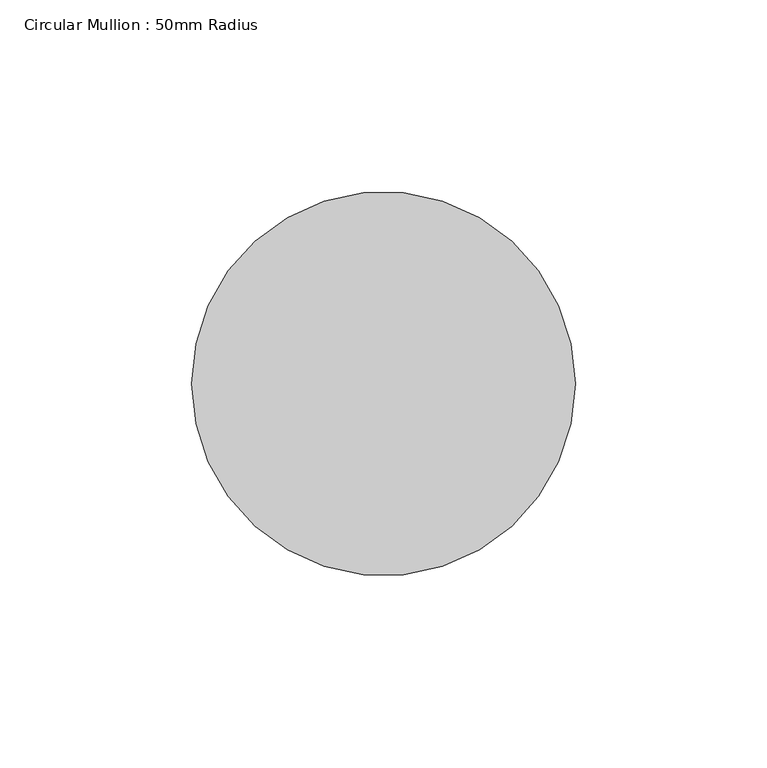
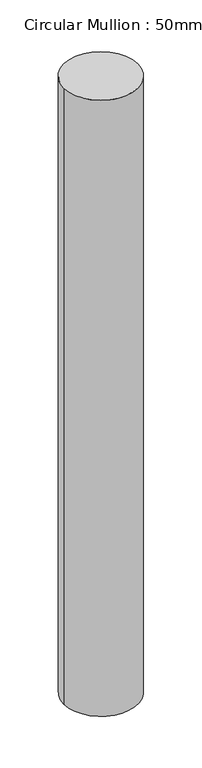
"""IFC4 building model written with IfcOpenShell, lengths in millimetres: member geometry, Circular Mullion : 50mm Radius."""

from ifc_helpers import new_model, si_unit, point, frame, origin, origin_2d, place, context, project, spatial, circle_curve, trimmed, segment, composite_curve, outline, extrude, source, transform, mapped, element, save


def circular_mullion_50mm_radius_d37bc5d8(model_context):
    return source(origin(), model_context, "Body", "SweptSolid", [
        extrude(outline(composite_curve([segment(trimmed(circle_curve(origin_2d(), 50.0), [point((50.0, 0.0))], [point((-50.0, 0.0))], False, "CARTESIAN"), True, "CONTINUOUS"), segment(trimmed(circle_curve(origin_2d(), 50.0), [point((-50.0, 0.0))], [point((50.0, 0.0))], False, "CARTESIAN"), True, "CONTINUOUS")], self_intersect=False)), frame((0.0, 0.0, -881.9892707), z_axis=(0.0, 0.0, 1.0), x_axis=(1.0, 0.0, 0.0)), (0.0, 0.0, 1.0), 881.9892707),
    ])


if __name__ == "__main__":
    model = new_model("IFC4")
    model_context = context("Model", 3, world=origin())
    ifc_project = project(units=[si_unit("LENGTHUNIT", "METRE", prefix="MILLI")], contexts=[model_context])
    site = spatial("IfcSite", under=ifc_project)
    building = spatial("IfcBuilding", under=site)
    placement = place(None, origin())
    circular_mullion_50mm_radius_shape = circular_mullion_50mm_radius_d37bc5d8(model_context)
    element("IfcMember", 1, ObjectType="Circular Mullion : 50mm Radius", at=placement, inside=building, context=model_context, shape_type="MappedRepresentation", body=[
        mapped(circular_mullion_50mm_radius_shape, transform((0.0, 0.0, 0.0), x_axis=(1.0, 0.0, 0.0), y_axis=(0.0, 1.0, 0.0), z_axis=(0.0, 0.0, 1.0))),
    ])
    save(model, "model.ifc")

# Revit data of these elements
# Type "Circular Mullion : 50mm Radius"
#   built-in parameter 1007350 = 0.164042 (stored number, unit not read)
# Element 1 (IfcMember, "Circular Mullion : 50mm Radius")
#   Materials on its faces: "Aluminium"
# Materials
#   "Aluminium": class "Metal", colour RGB 247 247 247, transparency 0, Description = "Aluminium 6061", Cost = 0
